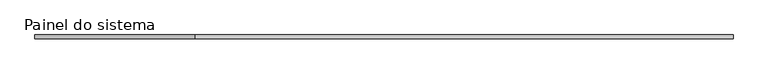
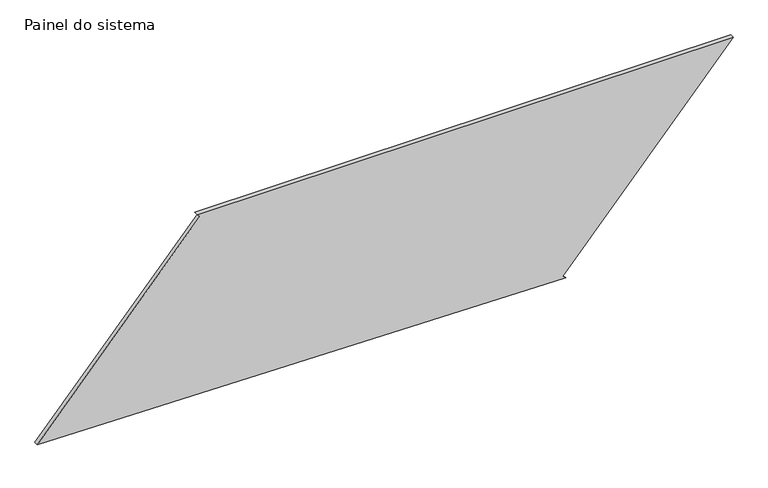
"""IFC4 building model written with IfcOpenShell, lengths in millimetres: plate geometry, Painel do sistema : Envidraçado."""

from ifc_helpers import new_model, si_unit, frame, origin, place, context, project, spatial, polyline, outline, extrude, source, transform, mapped, element, save


def painel_do_sistema_e87f30ce(model_context):
    return source(origin(), model_context, "Body", "SweptSolid", [
        extrude(outline(polyline([(0.0, 1143.3982573), (16.5356636, 1124.6480086), (1241.2425208, 2204.7051814), (1241.2425208, -1192.0883398), (1224.7068571, -1173.338091), (55.2110382, -2204.7051814), (0.0, 1143.3982573)])), frame((0.0, 24.5, 0.0), z_axis=(0.0, 1.0, 0.0), x_axis=(0.0, 0.0, 1.0)), (0.0, 0.0, 1.0), 25.0),
    ])


if __name__ == "__main__":
    model = new_model("IFC4")
    model_context = context("Model", 3, world=origin())
    ifc_project = project(units=[si_unit("LENGTHUNIT", "METRE", prefix="MILLI")], contexts=[model_context])
    site = spatial("IfcSite", under=ifc_project)
    building = spatial("IfcBuilding", under=site)
    placement = place(None, origin())
    painel_do_sistema_shape = painel_do_sistema_e87f30ce(model_context)
    element("IfcPlate", 1, ObjectType="Painel do sistema : Envidraçado", at=placement, inside=building, context=model_context, shape_type="MappedRepresentation", body=[
        mapped(painel_do_sistema_shape, transform((0.0, 0.0, 0.0), x_axis=(1.0, 0.0, 0.0), y_axis=(0.0, 1.0, 0.0), z_axis=(0.0, 0.0, 1.0))),
    ])
    save(model, "model.ifc")

# Revit data of these elements
# Type "Painel do sistema : Envidraçado"
#   Construction Type Id = "GSP4R"
#   Analytic Construction = "Vidraça única Pilkington 1/8 pol"
#   Visual Light Transmittance = 0.9
#   Solar Heat Gain Coefficient = 0.86
#   Heat Transfer Coefficient (U) = 6.7069 W/(m²·K)
# Element 1 (IfcPlate, "Painel do sistema : Envidraçado")
#   Materials on its faces: "Vidro"
# Materials
#   "Vidro": class "Vidro", colour RGB 0 128 192, transparency 0.9, Description = "Vidro de sílica", Cost = 0
